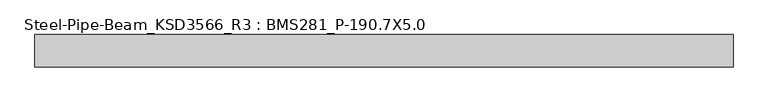
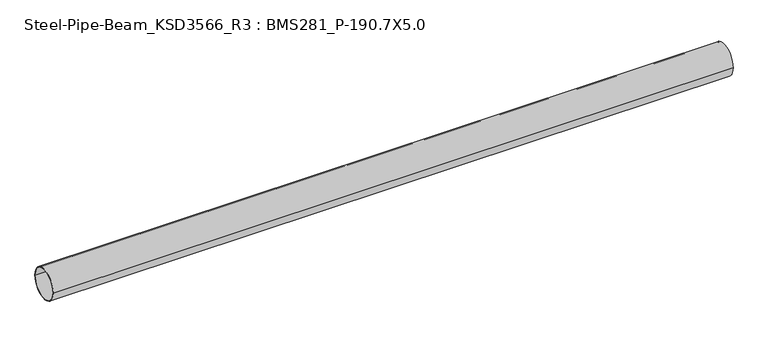
"""IFC4 building model written with IfcOpenShell, lengths in millimetres: member geometry, Steel-Pipe-Beam_KSD3566_R3 : BMS281_P-190.7X5.0."""

from ifc_helpers import new_model, si_unit, point, frame, origin, origin_2d, place, context, project, spatial, circle_curve, trimmed, segment, composite_curve, outline, extrude, source, transform, mapped, element, save


def steel_pipe_beam_ksd3566_r3_bms281_p_190_7x5_0_c465c395(model_context):
    return source(origin(), model_context, "Body", "SweptSolid", [
        extrude(outline(composite_curve([segment(trimmed(circle_curve(origin_2d(), 95.35), [point((-95.35, 0.0))], [point((95.35, 0.0))], False, "CARTESIAN"), True, "CONTINUOUS"), segment(trimmed(circle_curve(origin_2d(), 95.35), [point((95.35, 0.0))], [point((-95.35, 0.0))], False, "CARTESIAN"), True, "CONTINUOUS")], self_intersect=False), holes=[composite_curve([segment(trimmed(circle_curve(origin_2d(), 90.35), [point((90.35, 0.0))], [point((-90.35, 0.0))], True, "CARTESIAN"), True, "CONTINUOUS"), segment(trimmed(circle_curve(origin_2d(), 90.35), [point((-90.35, 0.0))], [point((90.35, 0.0))], True, "CARTESIAN"), True, "CONTINUOUS")], self_intersect=False)]), frame((-2046.1374086, 0.0, 0.0), z_axis=(1.0, 0.0, 0.0), x_axis=(0.0, 1.0, 0.0)), (0.0, 0.0, 1.0), 4105.6913247),
    ])


if __name__ == "__main__":
    model = new_model("IFC4")
    model_context = context("Model", 3, world=origin())
    ifc_project = project(units=[si_unit("LENGTHUNIT", "METRE", prefix="MILLI")], contexts=[model_context])
    site = spatial("IfcSite", under=ifc_project)
    building = spatial("IfcBuilding", under=site)
    placement = place(None, origin())
    steel_pipe_beam_ksd3566_r3_bms281_p_190_7x5_0_shape = steel_pipe_beam_ksd3566_r3_bms281_p_190_7x5_0_c465c395(model_context)
    element("IfcMember", 1, ObjectType="Steel-Pipe-Beam_KSD3566_R3 : BMS281_P-190.7X5.0", at=placement, inside=building, context=model_context, shape_type="MappedRepresentation", body=[
        mapped(steel_pipe_beam_ksd3566_r3_bms281_p_190_7x5_0_shape, transform((0.0, 0.0, 0.0), x_axis=(1.0, 0.0, 0.0), y_axis=(0.0, 1.0, 0.0), z_axis=(0.0, 0.0, 1.0))),
    ])
    save(model, "model.ifc")

# Revit data of these elements
# Type "Steel-Pipe-Beam_KSD3566_R3 : BMS281_P-190.7X5.0"
#   Keynote = "P-190.7X5.0"
#   SteelWeight = "Light"
#   t = 0.0050 m
#   Surface Area = 0.599102 m²/m
#   Section Area = 29.1697 cm²
#   Mass per Unit Length = 22.8982 kg/m
#   Length [instance default] = 1.5000 m
#   D = 0.1907 m
#   hec_material4 [instance default] = none
#   hec_material3 [instance default] = none
#   hec_material2 [instance default] = none
#   hec_material1 [instance default] = none
#   Structural Material [instance default] = Steel, 45-345
#   Assembly Code = ""
# Element 1 (IfcMember, "Steel-Pipe-Beam_KSD3566_R3 : BMS281_P-190.7X5.0")
#   Structural Material = none
# Materials
#   "Steel, 45-345": class "Metal", colour RGB 189 187 185, transparency 0, Description = "Steel 345 MPa", Cost = 0
